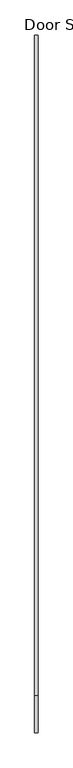
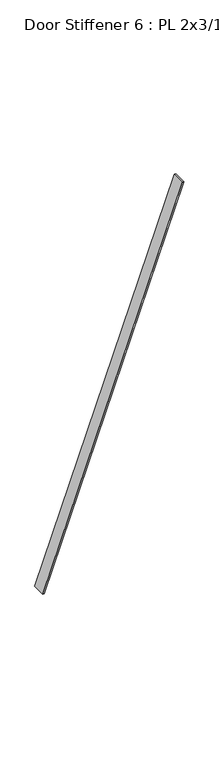
"""IFC4 building model written with IfcOpenShell, lengths in millimetres: proxy geometry, Door Stiffener 6 : PL 2x3/16."""

from ifc_helpers import new_model, si_unit, frame, origin, place, context, project, spatial, polyline, outline, extrude, source, transform, mapped, element, save


def door_stiffener_6_pl_2x3_16_59935e34(model_context):
    return source(origin(), model_context, "Body", "SweptSolid", [
        extrude(outline(polyline([(-536208.5749853, 2400.3), (-535246.0163841, 88.9), (-535301.0452829, 88.9), (-536263.6038841, 2400.3), (-536208.5749853, 2400.3)])), frame((587403.9934739, 0.0, 0.0), z_axis=(1.0, 0.0, 0.0), x_axis=(0.0, 1.0, 0.0)), (0.0, 0.0, 1.0), 4.7625),
    ])


if __name__ == "__main__":
    model = new_model("IFC4")
    model_context = context("Model", 3, world=origin())
    ifc_project = project(units=[si_unit("LENGTHUNIT", "METRE", prefix="MILLI")], contexts=[model_context])
    site = spatial("IfcSite", under=ifc_project)
    building = spatial("IfcBuilding", under=site)
    placement = place(None, origin())
    door_stiffener_6_pl_2x3_16_shape = door_stiffener_6_pl_2x3_16_59935e34(model_context)
    element("IfcBuildingElementProxy", 1, Name="Door Stiffener 6 : PL 2x3/16", ObjectType="Door Stiffener 6 : PL 2x3/16", at=placement, inside=building, context=model_context, shape_type="MappedRepresentation", body=[
        mapped(door_stiffener_6_pl_2x3_16_shape, transform((0.0, 0.0, 0.0), x_axis=(1.0, 0.0, 0.0), y_axis=(0.0, 1.0, 0.0), z_axis=(0.0, 0.0, 1.0))),
    ])
    save(model, "model.ifc")

# Revit data of these elements
# Element 1 (IfcBuildingElementProxy, "Door Stiffener 6 : PL 2x3/16")
#   Materials on its faces: "2\"X3/16\" GALV. STL BAR STOCK"
# Materials
#   "2\"X3/16\" GALV. STL BAR STOCK": class "Generic", colour RGB 211 211 207, transparency 0, Cost = 0
